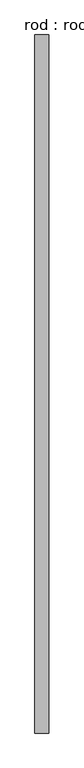
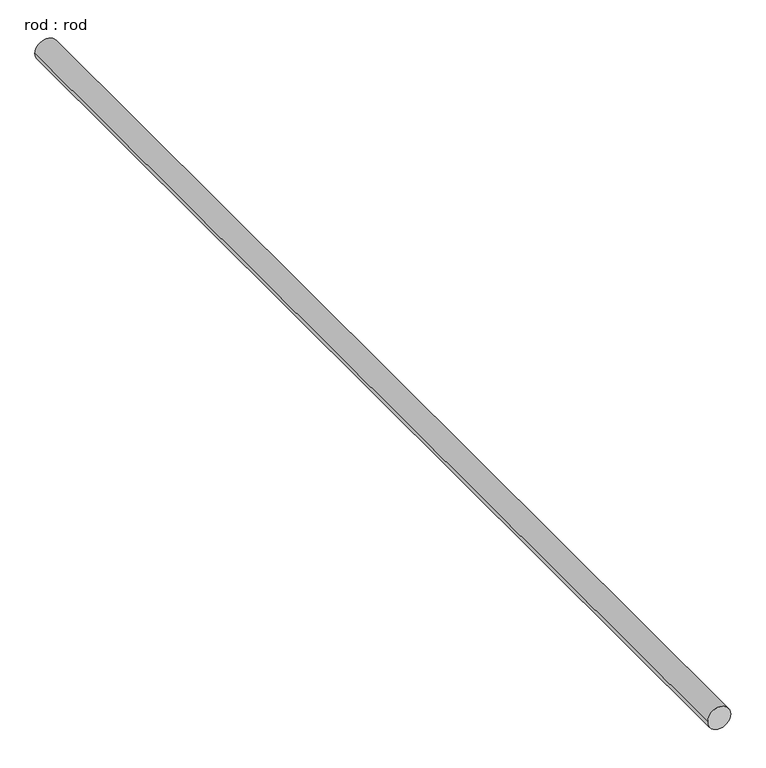
"""IFC4 building model written with IfcOpenShell, lengths in millimetres: proxy geometry, rod : rod."""

import ifcopenshell
import ifcopenshell.guid

model = None  # the IFC model being written
_history = None  # IfcOwnerHistory: only IFC2X3 demands one
_inside = {}  # id of a spatial element -> (the spatial element, [elements in it])
_under = {}  # id of a project, library or spatial element -> (it, [spatial elements below it])
_declared = {}  # id of a project -> (the project, [libraries it declares])
_typed = {}  # id of a type object -> (the type object, [elements of that type])
_made_of = {}  # id of a material, layer set ... -> (it, [elements and type objects made of it])


def new_model(schema):
    """Start an empty IFC model of exactly this schema.

    Asked for "IFC4X3", IfcOpenShell would pick the latest addendum, in which some entities
    have other attributes; the version numbers below select the first issue.
    IFC2X3 requires an IfcOwnerHistory on every rooted entity: one is made here for all.
    """
    global model, _history
    if schema == "IFC4X3":
        model = ifcopenshell.file(schema_version=(4, 3, 0, 0))
    else:
        model = ifcopenshell.file(schema=schema)
    _inside.clear()
    _under.clear()
    _declared.clear()
    _typed.clear()
    _made_of.clear()
    _history = None
    if model.schema == "IFC2X3":
        org = make("IfcOrganization", Name="unknown")
        user = make(
            "IfcPersonAndOrganization",
            ThePerson=make("IfcPerson", FamilyName="unknown"),
            TheOrganization=org,
        )
        app = make(
            "IfcApplication",
            ApplicationDeveloper=org,
            Version="unknown",
            ApplicationFullName="unknown",
            ApplicationIdentifier="unknown",
        )
        _history = make(
            "IfcOwnerHistory",
            OwningUser=user,
            OwningApplication=app,
            ChangeAction="ADDED",
            CreationDate=0,
        )
    return model


def make(cls, **values):
    """One entity of the class cls with the attributes given. An attribute that is None is left unset."""
    return model.create_entity(
        cls, **{name: value for name, value in values.items() if value is not None}
    )


def rooted(cls, **values):
    """An entity with a GlobalId (a new one), such as an element, a storey or a relation."""
    return make(cls, GlobalId=ifcopenshell.guid.new(), OwnerHistory=_history, **values)


def si_unit(unit_type, name, prefix=None):
    """IfcSIUnit, for example si_unit("LENGTHUNIT", "METRE", prefix="MILLI")."""
    return make("IfcSIUnit", UnitType=unit_type, Prefix=prefix, Name=name)


def assignment(units):
    """IfcUnitAssignment: the units of a project."""
    return None if units is None else make("IfcUnitAssignment", Units=units)


def point(xyz):
    """IfcCartesianPoint."""
    return None if xyz is None else make("IfcCartesianPoint", Coordinates=xyz)


def direction(xyz):
    """IfcDirection."""
    return None if xyz is None else make("IfcDirection", DirectionRatios=xyz)


def frame(location, z_axis=None, x_axis=None):
    """IfcAxis2Placement3D, a coordinate frame: its origin and axes. An axis left out is left unset."""
    return make(
        "IfcAxis2Placement3D",
        Location=point(location),
        Axis=direction(z_axis),
        RefDirection=direction(x_axis),
    )


def frame_2d(location, x_axis=None):
    """IfcAxis2Placement2D, a coordinate frame in the plane: its origin and x axis."""
    return make(
        "IfcAxis2Placement2D", Location=point(location), RefDirection=direction(x_axis)
    )


def origin():
    """The frame at (0, 0, 0) with its axes left unset."""
    return frame((0.0, 0.0, 0.0))


def place(relative_to, where):
    """IfcLocalPlacement: puts the frame where relative to a parent placement (None: the world)."""
    return make(
        "IfcLocalPlacement", PlacementRelTo=relative_to, RelativePlacement=where
    )


def context(
    kind, dimensions, precision=None, world=None, true_north=None, identifier=None
):
    """IfcGeometricRepresentationContext, for example the 3D "Model" context."""
    return make(
        "IfcGeometricRepresentationContext",
        ContextIdentifier=identifier,
        ContextType=kind,
        CoordinateSpaceDimension=dimensions,
        Precision=precision,
        WorldCoordinateSystem=world,
        TrueNorth=true_north,
    )


def project(units=None, contexts=None):
    """IfcProject with its units and contexts."""
    return rooted(
        "IfcProject",
        Name="project",
        RepresentationContexts=contexts,
        UnitsInContext=assignment(units),
    )


def spatial(cls, under=None, at=None, **own):
    """A site, building, storey or space (cls), placed at a placement, below another one or the project."""
    s = rooted(cls, ObjectPlacement=at, **own)
    if under is not None:
        _under.setdefault(under.id(), (under, []))[1].append(s)
    return s


def circle_curve(where, radius):
    """IfcCircle in the frame where."""
    return make("IfcCircle", Position=where, Radius=radius)


def trimmed(basis, trim1, trim2, sense, master):
    """IfcTrimmedCurve: the piece of a basis curve between two trims."""
    return make(
        "IfcTrimmedCurve",
        BasisCurve=basis,
        Trim1=trim1,
        Trim2=trim2,
        SenseAgreement=sense,
        MasterRepresentation=master,
    )


def segment(curve, same_sense, transition):
    """IfcCompositeCurveSegment."""
    return make(
        "IfcCompositeCurveSegment",
        Transition=transition,
        SameSense=same_sense,
        ParentCurve=curve,
    )


def composite_curve(segments, self_intersect=None):
    """IfcCompositeCurve: segments joined end to end."""
    return make("IfcCompositeCurve", Segments=segments, SelfIntersect=self_intersect)


def outline(outer, holes=None, kind="AREA"):
    """IfcArbitraryClosedProfileDef: a profile drawn as a closed curve; with holes, ...WithVoids."""
    if holes is None:
        return make("IfcArbitraryClosedProfileDef", ProfileType=kind, OuterCurve=outer)
    return make(
        "IfcArbitraryProfileDefWithVoids",
        ProfileType=kind,
        OuterCurve=outer,
        InnerCurves=holes,
    )


def extrude(swept, where, along, depth):
    """IfcExtrudedAreaSolid: the profile swept, set in the frame where, extruded along a direction by depth."""
    return make(
        "IfcExtrudedAreaSolid",
        SweptArea=swept,
        Position=where,
        ExtrudedDirection=direction(along),
        Depth=depth,
    )


def shape(context_of_items, identifier, shape_type, items):
    """IfcShapeRepresentation: the items that make up one representation, for example the "Body"."""
    return make(
        "IfcShapeRepresentation",
        ContextOfItems=context_of_items,
        RepresentationIdentifier=identifier,
        RepresentationType=shape_type,
        Items=items,
    )


def source(mapping_origin, context_of_items, identifier, shape_type, items):
    """IfcRepresentationMap: a shape defined once, which mapped items show again and again."""
    return make(
        "IfcRepresentationMap",
        MappingOrigin=mapping_origin,
        MappedRepresentation=shape(context_of_items, identifier, shape_type, items),
    )


def transform(
    local_origin,
    x_axis=None,
    y_axis=None,
    z_axis=None,
    scale=None,
    scale2=None,
    scale3=None,
    uniform=True,
):
    """IfcCartesianTransformationOperator3D, or its non-uniform kind. x_axis, y_axis, z_axis: its Axis1, 2, 3."""
    if uniform:
        return make(
            "IfcCartesianTransformationOperator3D",
            Axis1=direction(x_axis),
            Axis2=direction(y_axis),
            LocalOrigin=point(local_origin),
            Scale=scale,
            Axis3=direction(z_axis),
        )
    return make(
        "IfcCartesianTransformationOperator3DnonUniform",
        Axis1=direction(x_axis),
        Axis2=direction(y_axis),
        LocalOrigin=point(local_origin),
        Scale=scale,
        Axis3=direction(z_axis),
        Scale2=scale2,
        Scale3=scale3,
    )


def mapped(mapping_source, mapping_target):
    """IfcMappedItem: shows the shape of a source again, moved by a transform."""
    return make(
        "IfcMappedItem", MappingSource=mapping_source, MappingTarget=mapping_target
    )


def made_of(thing, what):
    """Note that an element or type object is made of a material, layer set ...; save() writes the relation."""
    if what is not None:
        _made_of.setdefault(what.id(), (what, []))[1].append(thing)
    return thing


def element(
    cls,
    number,
    at=None,
    inside=None,
    cuts=None,
    type_object=None,
    material=None,
    context=None,
    identifier="Body",
    shape_type=None,
    held_by="IfcProductDefinitionShape",
    body=None,
    shapes=None,
    **own,
):
    """One element of the class cls, such as IfcWall. Its Tag is "e" and its number.

    at: its placement. inside: the storey or other place that contains it. cuts: it is an
    opening in that element (IfcRelVoidsElement). A single representation is given by context,
    identifier, shape_type and body (its items); several are given by shapes. held_by: the class
    of the entity that holds the representations. save() writes the other relations.
    """
    e = rooted(cls, Tag="e%d" % number, ObjectPlacement=at, **own)
    if body is not None:
        shapes = [shape(context, identifier, shape_type, body)]
    if shapes is not None:
        e.Representation = make(held_by, Representations=shapes)
    if inside is not None:
        _inside.setdefault(inside.id(), (inside, []))[1].append(e)
    if cuts is not None:
        rooted(
            "IfcRelVoidsElement", RelatingBuildingElement=cuts, RelatedOpeningElement=e
        )
    if type_object is not None:
        _typed.setdefault(type_object.id(), (type_object, []))[1].append(e)
    return made_of(e, material)


def aggregate(whole, parts):
    """IfcRelAggregates: a whole, such as a stair, and the parts it consists of."""
    return rooted("IfcRelAggregates", RelatingObject=whole, RelatedObjects=parts)


def save(model, path):
    """Write the relations noted so far, then the file.

    IfcRelAggregates (storeys below a building ...), IfcRelContainedInSpatialStructure (elements
    in a storey), IfcRelDefinesByType, IfcRelAssociatesMaterial and IfcRelDeclares: one each for
    every whole, place, type object, material and project.
    """
    for whole, parts in _under.values():
        aggregate(whole, parts)
    for where, things in _inside.values():
        rooted(
            "IfcRelContainedInSpatialStructure",
            RelatedElements=things,
            RelatingStructure=where,
        )
    for kind, things in _typed.values():
        rooted("IfcRelDefinesByType", RelatedObjects=things, RelatingType=kind)
    for what, things in _made_of.values():
        rooted("IfcRelAssociatesMaterial", RelatedObjects=things, RelatingMaterial=what)
    for by, libraries in _declared.values():
        rooted("IfcRelDeclares", RelatingContext=by, RelatedDefinitions=libraries)
    model.write(path)


def rod_rod_716b9a16(model_context):
    return source(origin(), model_context, "Body", "SweptSolid", [
        extrude(outline(composite_curve([segment(trimmed(circle_curve(frame_2d((0.0108462, 0.0)), 200.0), [point((0.0108462, 200.0))], [point((0.0108462, -200.0))], False, "CARTESIAN"), True, "CONTINUOUS"), segment(trimmed(circle_curve(frame_2d((0.0108462, 0.0)), 200.0), [point((0.0108462, -200.0))], [point((0.0108462, 200.0))], False, "CARTESIAN"), True, "CONTINUOUS")], self_intersect=False)), frame((0.0, -6012.19871, 0.0), z_axis=(0.0, 1.0, 0.0), x_axis=(0.0, 0.0, 1.0)), (0.0, 0.0, 1.0), 20209.8546506),
    ])


if __name__ == "__main__":
    model = new_model("IFC4")
    model_context = context("Model", 3, world=origin())
    ifc_project = project(units=[si_unit("LENGTHUNIT", "METRE", prefix="MILLI")], contexts=[model_context])
    site = spatial("IfcSite", under=ifc_project)
    building = spatial("IfcBuilding", under=site)
    placement = place(None, origin())
    rod_rod_shape = rod_rod_716b9a16(model_context)
    element("IfcBuildingElementProxy", 1, Name="rod : rod", ObjectType="rod : rod", at=placement, inside=building, context=model_context, shape_type="MappedRepresentation", body=[
        mapped(rod_rod_shape, transform((0.0, 0.0, 0.0), x_axis=(1.0, 0.0, 0.0), y_axis=(0.0, 1.0, 0.0), z_axis=(0.0, 0.0, 1.0))),
    ])
    save(model, "model.ifc")

# Revit data of these elements
# Type "rod : rod"
#   Default Elevation = 0
